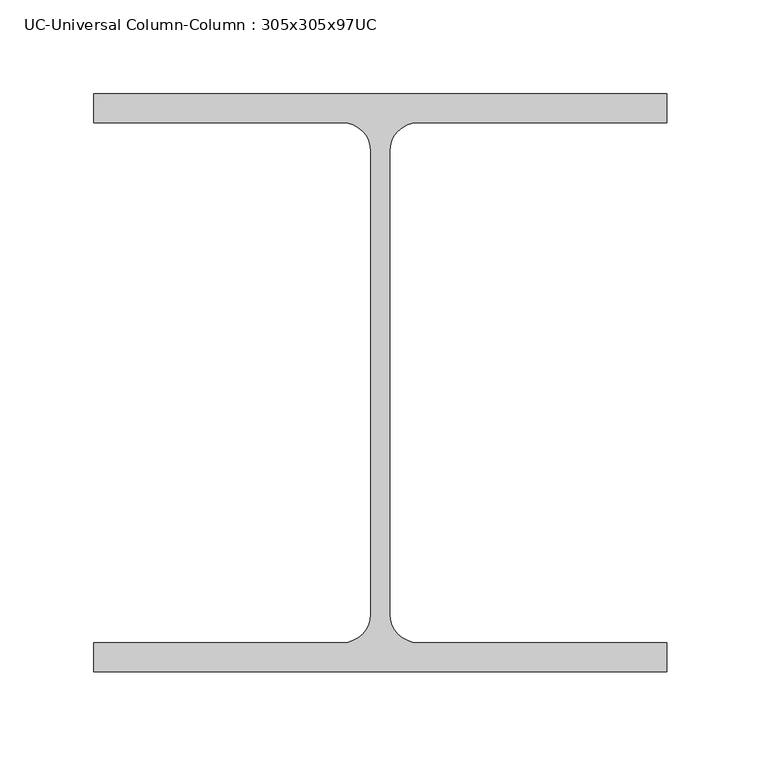
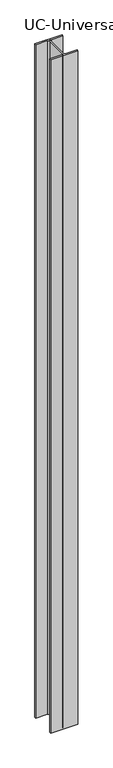
"""IFC4 building model written with IfcOpenShell, lengths in millimetres: column geometry, UC-Universal Column-Column : 305x305x97UC."""

import ifcopenshell
import ifcopenshell.guid

model = None  # the IFC model being written
_history = None  # IfcOwnerHistory: only IFC2X3 demands one
_inside = {}  # id of a spatial element -> (the spatial element, [elements in it])
_under = {}  # id of a project, library or spatial element -> (it, [spatial elements below it])
_declared = {}  # id of a project -> (the project, [libraries it declares])
_typed = {}  # id of a type object -> (the type object, [elements of that type])
_made_of = {}  # id of a material, layer set ... -> (it, [elements and type objects made of it])


def new_model(schema):
    """Start an empty IFC model of exactly this schema.

    Asked for "IFC4X3", IfcOpenShell would pick the latest addendum, in which some entities
    have other attributes; the version numbers below select the first issue.
    IFC2X3 requires an IfcOwnerHistory on every rooted entity: one is made here for all.
    """
    global model, _history
    if schema == "IFC4X3":
        model = ifcopenshell.file(schema_version=(4, 3, 0, 0))
    else:
        model = ifcopenshell.file(schema=schema)
    _inside.clear()
    _under.clear()
    _declared.clear()
    _typed.clear()
    _made_of.clear()
    _history = None
    if model.schema == "IFC2X3":
        org = make("IfcOrganization", Name="unknown")
        user = make(
            "IfcPersonAndOrganization",
            ThePerson=make("IfcPerson", FamilyName="unknown"),
            TheOrganization=org,
        )
        app = make(
            "IfcApplication",
            ApplicationDeveloper=org,
            Version="unknown",
            ApplicationFullName="unknown",
            ApplicationIdentifier="unknown",
        )
        _history = make(
            "IfcOwnerHistory",
            OwningUser=user,
            OwningApplication=app,
            ChangeAction="ADDED",
            CreationDate=0,
        )
    return model


def make(cls, **values):
    """One entity of the class cls with the attributes given. An attribute that is None is left unset."""
    return model.create_entity(
        cls, **{name: value for name, value in values.items() if value is not None}
    )


def rooted(cls, **values):
    """An entity with a GlobalId (a new one), such as an element, a storey or a relation."""
    return make(cls, GlobalId=ifcopenshell.guid.new(), OwnerHistory=_history, **values)


def si_unit(unit_type, name, prefix=None):
    """IfcSIUnit, for example si_unit("LENGTHUNIT", "METRE", prefix="MILLI")."""
    return make("IfcSIUnit", UnitType=unit_type, Prefix=prefix, Name=name)


def assignment(units):
    """IfcUnitAssignment: the units of a project."""
    return None if units is None else make("IfcUnitAssignment", Units=units)


def point(xyz):
    """IfcCartesianPoint."""
    return None if xyz is None else make("IfcCartesianPoint", Coordinates=xyz)


def direction(xyz):
    """IfcDirection."""
    return None if xyz is None else make("IfcDirection", DirectionRatios=xyz)


def frame(location, z_axis=None, x_axis=None):
    """IfcAxis2Placement3D, a coordinate frame: its origin and axes. An axis left out is left unset."""
    return make(
        "IfcAxis2Placement3D",
        Location=point(location),
        Axis=direction(z_axis),
        RefDirection=direction(x_axis),
    )


def frame_2d(location, x_axis=None):
    """IfcAxis2Placement2D, a coordinate frame in the plane: its origin and x axis."""
    return make(
        "IfcAxis2Placement2D", Location=point(location), RefDirection=direction(x_axis)
    )


def origin():
    """The frame at (0, 0, 0) with its axes left unset."""
    return frame((0.0, 0.0, 0.0))


def origin_with_axes():
    """The frame at (0, 0, 0) with the z axis (0, 0, 1) and the x axis (1, 0, 0) written out."""
    return frame((0.0, 0.0, 0.0), z_axis=(0.0, 0.0, 1.0), x_axis=(1.0, 0.0, 0.0))


def place(relative_to, where):
    """IfcLocalPlacement: puts the frame where relative to a parent placement (None: the world)."""
    return make(
        "IfcLocalPlacement", PlacementRelTo=relative_to, RelativePlacement=where
    )


def context(
    kind, dimensions, precision=None, world=None, true_north=None, identifier=None
):
    """IfcGeometricRepresentationContext, for example the 3D "Model" context."""
    return make(
        "IfcGeometricRepresentationContext",
        ContextIdentifier=identifier,
        ContextType=kind,
        CoordinateSpaceDimension=dimensions,
        Precision=precision,
        WorldCoordinateSystem=world,
        TrueNorth=true_north,
    )


def project(units=None, contexts=None):
    """IfcProject with its units and contexts."""
    return rooted(
        "IfcProject",
        Name="project",
        RepresentationContexts=contexts,
        UnitsInContext=assignment(units),
    )


def spatial(cls, under=None, at=None, **own):
    """A site, building, storey or space (cls), placed at a placement, below another one or the project."""
    s = rooted(cls, ObjectPlacement=at, **own)
    if under is not None:
        _under.setdefault(under.id(), (under, []))[1].append(s)
    return s


def polyline(points):
    """IfcPolyline through the points."""
    return make("IfcPolyline", Points=[point(p) for p in points])


def circle_curve(where, radius):
    """IfcCircle in the frame where."""
    return make("IfcCircle", Position=where, Radius=radius)


def trimmed(basis, trim1, trim2, sense, master):
    """IfcTrimmedCurve: the piece of a basis curve between two trims."""
    return make(
        "IfcTrimmedCurve",
        BasisCurve=basis,
        Trim1=trim1,
        Trim2=trim2,
        SenseAgreement=sense,
        MasterRepresentation=master,
    )


def segment(curve, same_sense, transition):
    """IfcCompositeCurveSegment."""
    return make(
        "IfcCompositeCurveSegment",
        Transition=transition,
        SameSense=same_sense,
        ParentCurve=curve,
    )


def composite_curve(segments, self_intersect=None):
    """IfcCompositeCurve: segments joined end to end."""
    return make("IfcCompositeCurve", Segments=segments, SelfIntersect=self_intersect)


def outline(outer, holes=None, kind="AREA"):
    """IfcArbitraryClosedProfileDef: a profile drawn as a closed curve; with holes, ...WithVoids."""
    if holes is None:
        return make("IfcArbitraryClosedProfileDef", ProfileType=kind, OuterCurve=outer)
    return make(
        "IfcArbitraryProfileDefWithVoids",
        ProfileType=kind,
        OuterCurve=outer,
        InnerCurves=holes,
    )


def extrude(swept, where, along, depth):
    """IfcExtrudedAreaSolid: the profile swept, set in the frame where, extruded along a direction by depth."""
    return make(
        "IfcExtrudedAreaSolid",
        SweptArea=swept,
        Position=where,
        ExtrudedDirection=direction(along),
        Depth=depth,
    )


def shape(context_of_items, identifier, shape_type, items):
    """IfcShapeRepresentation: the items that make up one representation, for example the "Body"."""
    return make(
        "IfcShapeRepresentation",
        ContextOfItems=context_of_items,
        RepresentationIdentifier=identifier,
        RepresentationType=shape_type,
        Items=items,
    )


def source(mapping_origin, context_of_items, identifier, shape_type, items):
    """IfcRepresentationMap: a shape defined once, which mapped items show again and again."""
    return make(
        "IfcRepresentationMap",
        MappingOrigin=mapping_origin,
        MappedRepresentation=shape(context_of_items, identifier, shape_type, items),
    )


def transform(
    local_origin,
    x_axis=None,
    y_axis=None,
    z_axis=None,
    scale=None,
    scale2=None,
    scale3=None,
    uniform=True,
):
    """IfcCartesianTransformationOperator3D, or its non-uniform kind. x_axis, y_axis, z_axis: its Axis1, 2, 3."""
    if uniform:
        return make(
            "IfcCartesianTransformationOperator3D",
            Axis1=direction(x_axis),
            Axis2=direction(y_axis),
            LocalOrigin=point(local_origin),
            Scale=scale,
            Axis3=direction(z_axis),
        )
    return make(
        "IfcCartesianTransformationOperator3DnonUniform",
        Axis1=direction(x_axis),
        Axis2=direction(y_axis),
        LocalOrigin=point(local_origin),
        Scale=scale,
        Axis3=direction(z_axis),
        Scale2=scale2,
        Scale3=scale3,
    )


def mapped(mapping_source, mapping_target):
    """IfcMappedItem: shows the shape of a source again, moved by a transform."""
    return make(
        "IfcMappedItem", MappingSource=mapping_source, MappingTarget=mapping_target
    )


def made_of(thing, what):
    """Note that an element or type object is made of a material, layer set ...; save() writes the relation."""
    if what is not None:
        _made_of.setdefault(what.id(), (what, []))[1].append(thing)
    return thing


def element(
    cls,
    number,
    at=None,
    inside=None,
    cuts=None,
    type_object=None,
    material=None,
    context=None,
    identifier="Body",
    shape_type=None,
    held_by="IfcProductDefinitionShape",
    body=None,
    shapes=None,
    **own,
):
    """One element of the class cls, such as IfcWall. Its Tag is "e" and its number.

    at: its placement. inside: the storey or other place that contains it. cuts: it is an
    opening in that element (IfcRelVoidsElement). A single representation is given by context,
    identifier, shape_type and body (its items); several are given by shapes. held_by: the class
    of the entity that holds the representations. save() writes the other relations.
    """
    e = rooted(cls, Tag="e%d" % number, ObjectPlacement=at, **own)
    if body is not None:
        shapes = [shape(context, identifier, shape_type, body)]
    if shapes is not None:
        e.Representation = make(held_by, Representations=shapes)
    if inside is not None:
        _inside.setdefault(inside.id(), (inside, []))[1].append(e)
    if cuts is not None:
        rooted(
            "IfcRelVoidsElement", RelatingBuildingElement=cuts, RelatedOpeningElement=e
        )
    if type_object is not None:
        _typed.setdefault(type_object.id(), (type_object, []))[1].append(e)
    return made_of(e, material)


def aggregate(whole, parts):
    """IfcRelAggregates: a whole, such as a stair, and the parts it consists of."""
    return rooted("IfcRelAggregates", RelatingObject=whole, RelatedObjects=parts)


def save(model, path):
    """Write the relations noted so far, then the file.

    IfcRelAggregates (storeys below a building ...), IfcRelContainedInSpatialStructure (elements
    in a storey), IfcRelDefinesByType, IfcRelAssociatesMaterial and IfcRelDeclares: one each for
    every whole, place, type object, material and project.
    """
    for whole, parts in _under.values():
        aggregate(whole, parts)
    for where, things in _inside.values():
        rooted(
            "IfcRelContainedInSpatialStructure",
            RelatedElements=things,
            RelatingStructure=where,
        )
    for kind, things in _typed.values():
        rooted("IfcRelDefinesByType", RelatedObjects=things, RelatingType=kind)
    for what, things in _made_of.values():
        rooted("IfcRelAssociatesMaterial", RelatedObjects=things, RelatingMaterial=what)
    for by, libraries in _declared.values():
        rooted("IfcRelDeclares", RelatingContext=by, RelatedDefinitions=libraries)
    model.write(path)


def uc_universal_column_column_305x305x97uc_b32ae94d(model_context):
    return source(origin(), model_context, "Body", "SweptSolid", [
        extrude(outline(composite_curve([segment(polyline([(152.65, 153.95), (152.65, 138.55), (20.15, 138.55)]), True, "CONTINUOUS"), segment(trimmed(circle_curve(frame_2d((20.15, 123.35)), 15.2), [point((20.15, 138.55))], [point((4.95, 123.35))], True, "CARTESIAN"), True, "CONTINUOUS"), segment(polyline([(4.95, 123.35), (4.95, -123.35)]), True, "CONTINUOUS"), segment(trimmed(circle_curve(frame_2d((20.15, -123.35)), 15.2), [point((4.95, -123.35))], [point((20.15, -138.55))], True, "CARTESIAN"), True, "CONTINUOUS"), segment(polyline([(20.15, -138.55), (152.65, -138.55), (152.65, -153.95), (-152.65, -153.95), (-152.65, -138.55), (-20.15, -138.55)]), True, "CONTINUOUS"), segment(trimmed(circle_curve(frame_2d((-20.15, -123.35)), 15.2), [point((-20.15, -138.55))], [point((-4.95, -123.35))], True, "CARTESIAN"), True, "CONTINUOUS"), segment(polyline([(-4.95, -123.35), (-4.95, 123.35)]), True, "CONTINUOUS"), segment(trimmed(circle_curve(frame_2d((-20.15, 123.35)), 15.2), [point((-4.95, 123.35))], [point((-20.15, 138.55))], True, "CARTESIAN"), True, "CONTINUOUS"), segment(polyline([(-20.15, 138.55), (-152.65, 138.55), (-152.65, 153.95), (152.65, 153.95)]), True, "CONTINUOUS")], self_intersect=False)), origin_with_axes(), (0.0, 0.0, 1.0), 8000.0),
    ])


if __name__ == "__main__":
    model = new_model("IFC4")
    model_context = context("Model", 3, world=origin())
    ifc_project = project(units=[si_unit("LENGTHUNIT", "METRE", prefix="MILLI")], contexts=[model_context])
    site = spatial("IfcSite", under=ifc_project)
    building = spatial("IfcBuilding", under=site)
    placement = place(None, origin())
    uc_universal_column_column_305x305x97uc_shape = uc_universal_column_column_305x305x97uc_b32ae94d(model_context)
    element("IfcColumn", 1, ObjectType="UC-Universal Column-Column : 305x305x97UC", at=placement, inside=building, context=model_context, shape_type="MappedRepresentation", body=[
        mapped(uc_universal_column_column_305x305x97uc_shape, transform((0.0, 0.0, 0.0), x_axis=(1.0, 0.0, 0.0), y_axis=(0.0, 1.0, 0.0), z_axis=(0.0, 0.0, 1.0))),
    ])
    save(model, "model.ifc")

# Revit data of these elements
# Type "UC-Universal Column-Column : 305x305x97UC"
#   Nominal h = "305"
#   W = 0
#   Ix = 22250
#   M = 96.9
#   Zx = 1445
#   b = 305.3 mm
#   h = 307.9 mm
#   r = 15.2 mm
#   s = 9.9 mm
#   t = 15.4 mm
#   A = 0.0123 m²
#   Structural Material [instance default] = Metal - Steel - 345 MPa
#   Assembly Code = ""
# Element 1 (IfcColumn, "UC-Universal Column-Column : 305x305x97UC")
#   Materials on its faces: "Metal - Steel - 345 MPa"
# Materials
#   "Metal - Steel - 345 MPa": class "Metal", colour RGB 241 46 46, transparency 0
